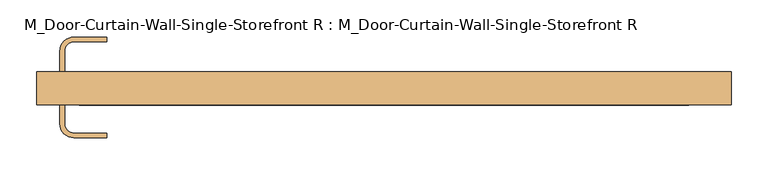
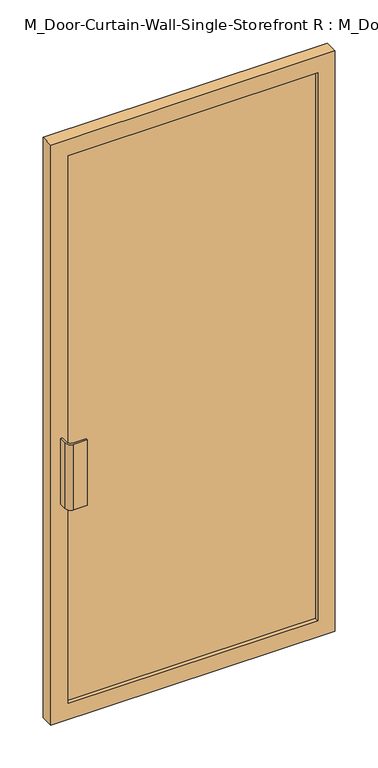
"""IFC4 building model written with IfcOpenShell, lengths in millimetres: door geometry, M_Door-Curtain-Wall-Single-Storefront R : M_Door-Curtain-Wall-Single-Storefront R."""

from ifc_helpers import new_model, si_unit, point, frame, frame_2d, origin, place, context, project, spatial, polyline, circle_curve, trimmed, segment, composite_curve, outline, extrude, source, transform, mapped, element, save


def m_door_curtain_wall_single_storefront_r_m_door_curtain_wall_a1f74e57(model_context):
    return source(origin(), model_context, "Body", "SweptSolid", [
        extrude(outline(polyline([(2025.65, -469.10625), (0.0, -469.10625), (0.0, 469.9), (2025.65, 469.9), (2025.65, -469.10625)]), holes=[polyline([(1968.5, -411.95625), (1968.5, 412.75), (57.15, 412.75), (57.15, -411.95625), (1968.5, -411.95625)])]), frame((0.0, -60.0, 0.0), z_axis=(0.0, 1.0, 0.0), x_axis=(0.0, 0.0, 1.0)), (0.0, 0.0, 1.0), 44.45),
        extrude(outline(polyline([(412.75, -28.25), (412.75, -47.3), (-411.95625, -47.3), (-411.95625, -28.25), (412.75, -28.25)])), frame((0.0, 0.0, 57.15), z_axis=(0.0, 0.0, 1.0), x_axis=(1.0, 0.0, 0.0)), (0.0, 0.0, 1.0), 1911.35),
        extrude(outline(composite_curve([segment(trimmed(circle_curve(frame_2d((-419.1, 12.7)), 19.05), [point((-438.15, 12.7))], [point((-419.1, 31.75))], False, "CARTESIAN"), True, "CONTINUOUS"), segment(polyline([(-419.1, 31.75), (-374.65, 31.75), (-374.65, 25.4), (-419.1, 25.4)]), True, "CONTINUOUS"), segment(trimmed(circle_curve(frame_2d((-419.1, 12.7)), 12.7), [point((-419.1, 25.4))], [point((-431.8, 12.7))], True, "CARTESIAN"), True, "CONTINUOUS"), segment(polyline([(-431.8, 12.7), (-431.8, -15.55), (-438.15, -15.55), (-438.15, 12.7)]), True, "CONTINUOUS")], self_intersect=False)), frame((0.0, 0.0, 762.0), z_axis=(0.0, 0.0, 1.0), x_axis=(1.0, 0.0, 0.0)), (0.0, 0.0, 1.0), 228.6),
        extrude(outline(composite_curve([segment(polyline([(-438.15, -85.4), (-438.15, -60.0), (-431.8, -60.0), (-431.8, -85.4)]), True, "CONTINUOUS"), segment(trimmed(circle_curve(frame_2d((-419.1, -85.4)), 12.7), [point((-431.8, -85.4))], [point((-419.1, -98.1))], True, "CARTESIAN"), True, "CONTINUOUS"), segment(polyline([(-419.1, -98.1), (-374.65, -98.1), (-374.65, -104.45), (-419.1, -104.45)]), True, "CONTINUOUS"), segment(trimmed(circle_curve(frame_2d((-419.1, -85.4)), 19.05), [point((-419.1, -104.45))], [point((-438.15, -85.4))], False, "CARTESIAN"), True, "CONTINUOUS")], self_intersect=False)), frame((0.0, 0.0, 762.0), z_axis=(0.0, 0.0, 1.0), x_axis=(1.0, 0.0, 0.0)), (0.0, 0.0, 1.0), 228.6),
    ])


if __name__ == "__main__":
    model = new_model("IFC4")
    model_context = context("Model", 3, world=origin())
    ifc_project = project(units=[si_unit("LENGTHUNIT", "METRE", prefix="MILLI")], contexts=[model_context])
    site = spatial("IfcSite", under=ifc_project)
    building = spatial("IfcBuilding", under=site)
    placement = place(None, origin())
    m_door_curtain_wall_single_storefront_r_m_door_curtain_wall_shape = m_door_curtain_wall_single_storefront_r_m_door_curtain_wall_a1f74e57(model_context)
    element("IfcDoor", 1, ObjectType="M_Door-Curtain-Wall-Single-Storefront R : M_Door-Curtain-Wall-Single-Storefront R", at=placement, inside=building, context=model_context, shape_type="MappedRepresentation", body=[
        mapped(m_door_curtain_wall_single_storefront_r_m_door_curtain_wall_shape, transform((0.0, 0.0, 0.0), x_axis=(1.0, 0.0, 0.0), y_axis=(0.0, 1.0, 0.0), z_axis=(0.0, 0.0, 1.0))),
    ])
    save(model, "model.ifc")

# Revit data of these elements
# Type "M_Door-Curtain-Wall-Single-Storefront R : M_Door-Curtain-Wall-Single-Storefront R"
#   Type Mark = "d"
#   Construction Type Id = "opn-d46"
#   Assembly Code = "B2030100"
#   Analytic Construction = "Metal frame, double glass door"
#   Width [instance default] = 5' - 10.86614"
#   Thermal Resistance (R) = 0.242926 (m²·K)/W
#   Swing Angle [instance default] = 90.00°
#   Offset = 0' - 2.3622"
#   Heat Transfer Coefficient (U) = 4.11674 W/(m²·K)
#   Function = 1
#   Frame Material = Aluminum
#   Door Handle Material = Aluminum
#   Glazing = EXISTING WINDOW
#   Visual Light Transmittance = 0
#   Solar Heat Gain Coefficient = 0
# Element 1 (IfcDoor, "M_Door-Curtain-Wall-Single-Storefront R : M_Door-Curtain-Wall-Single-Storefront R")
#   Materials on its faces: "Aluminum", "EXISTING WINDOW"
# Materials
#   "Aluminum": class "Metal", colour RGB 244 244 244, transparency 0, Description = "Aluminum 6061", Cost = 0
#   "EXISTING WINDOW": class "Glass", colour RGB 218 227 224, transparency 0.85, Description = "Soda Lime Glass", Cost = 0
